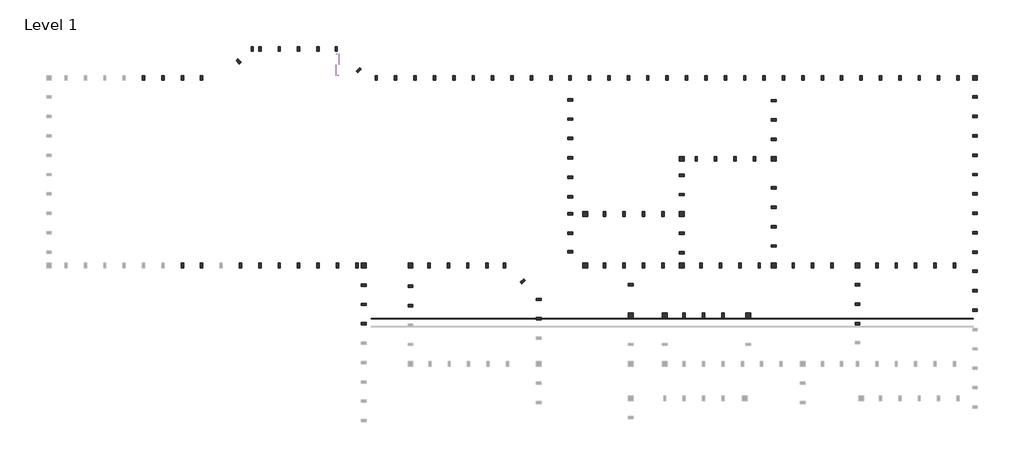
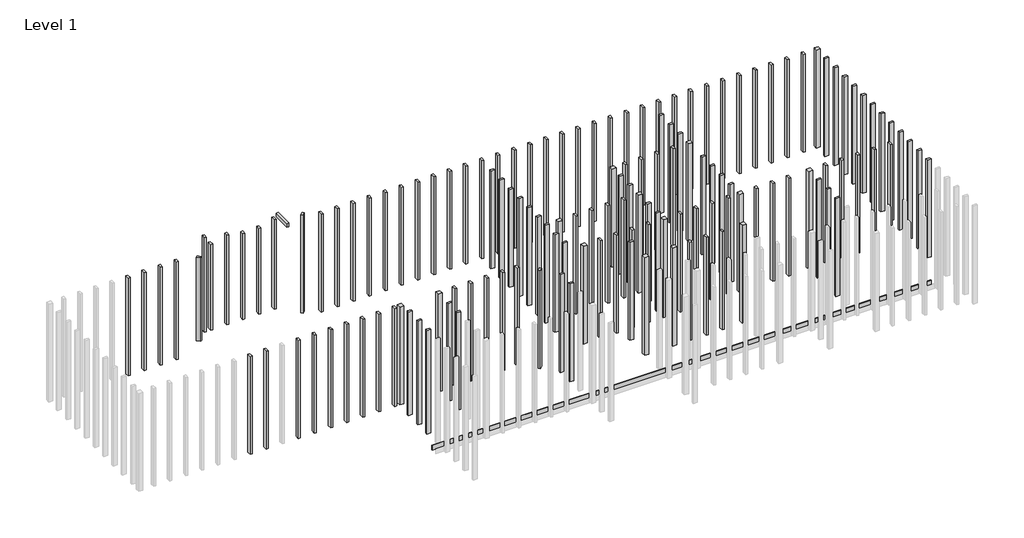
# One storey, part 2 of 2: 142 columns, 3 beams.
"""IFC4 building model written with IfcOpenShell, lengths in millimetres."""

import ifcopenshell
import ifcopenshell.guid

model = None  # the IFC model being written
_history = None  # IfcOwnerHistory: only IFC2X3 demands one
_inside = {}  # id of a spatial element -> (the spatial element, [elements in it])
_under = {}  # id of a project, library or spatial element -> (it, [spatial elements below it])
_declared = {}  # id of a project -> (the project, [libraries it declares])
_typed = {}  # id of a type object -> (the type object, [elements of that type])
_made_of = {}  # id of a material, layer set ... -> (it, [elements and type objects made of it])


def new_model(schema):
    """Start an empty IFC model of exactly this schema.

    Asked for "IFC4X3", IfcOpenShell would pick the latest addendum, in which some entities
    have other attributes; the version numbers below select the first issue.
    IFC2X3 requires an IfcOwnerHistory on every rooted entity: one is made here for all.
    """
    global model, _history
    if schema == "IFC4X3":
        model = ifcopenshell.file(schema_version=(4, 3, 0, 0))
    else:
        model = ifcopenshell.file(schema=schema)
    _inside.clear()
    _under.clear()
    _declared.clear()
    _typed.clear()
    _made_of.clear()
    _history = None
    if model.schema == "IFC2X3":
        org = make("IfcOrganization", Name="unknown")
        user = make(
            "IfcPersonAndOrganization",
            ThePerson=make("IfcPerson", FamilyName="unknown"),
            TheOrganization=org,
        )
        app = make(
            "IfcApplication",
            ApplicationDeveloper=org,
            Version="unknown",
            ApplicationFullName="unknown",
            ApplicationIdentifier="unknown",
        )
        _history = make(
            "IfcOwnerHistory",
            OwningUser=user,
            OwningApplication=app,
            ChangeAction="ADDED",
            CreationDate=0,
        )
    return model


def make(cls, **values):
    """One entity of the class cls with the attributes given. An attribute that is None is left unset."""
    return model.create_entity(
        cls, **{name: value for name, value in values.items() if value is not None}
    )


def rooted(cls, **values):
    """An entity with a GlobalId (a new one), such as an element, a storey or a relation."""
    return make(cls, GlobalId=ifcopenshell.guid.new(), OwnerHistory=_history, **values)


def si_unit(unit_type, name, prefix=None):
    """IfcSIUnit, for example si_unit("LENGTHUNIT", "METRE", prefix="MILLI")."""
    return make("IfcSIUnit", UnitType=unit_type, Prefix=prefix, Name=name)


def assignment(units):
    """IfcUnitAssignment: the units of a project."""
    return None if units is None else make("IfcUnitAssignment", Units=units)


def point(xyz):
    """IfcCartesianPoint."""
    return None if xyz is None else make("IfcCartesianPoint", Coordinates=xyz)


def direction(xyz):
    """IfcDirection."""
    return None if xyz is None else make("IfcDirection", DirectionRatios=xyz)


def frame(location, z_axis=None, x_axis=None):
    """IfcAxis2Placement3D, a coordinate frame: its origin and axes. An axis left out is left unset."""
    return make(
        "IfcAxis2Placement3D",
        Location=point(location),
        Axis=direction(z_axis),
        RefDirection=direction(x_axis),
    )


def origin():
    """The frame at (0, 0, 0) with its axes left unset."""
    return frame((0.0, 0.0, 0.0))


def origin_with_axes():
    """The frame at (0, 0, 0) with the z axis (0, 0, 1) and the x axis (1, 0, 0) written out."""
    return frame((0.0, 0.0, 0.0), z_axis=(0.0, 0.0, 1.0), x_axis=(1.0, 0.0, 0.0))


def place(relative_to, where):
    """IfcLocalPlacement: puts the frame where relative to a parent placement (None: the world)."""
    return make(
        "IfcLocalPlacement", PlacementRelTo=relative_to, RelativePlacement=where
    )


def context(
    kind, dimensions, precision=None, world=None, true_north=None, identifier=None
):
    """IfcGeometricRepresentationContext, for example the 3D "Model" context."""
    return make(
        "IfcGeometricRepresentationContext",
        ContextIdentifier=identifier,
        ContextType=kind,
        CoordinateSpaceDimension=dimensions,
        Precision=precision,
        WorldCoordinateSystem=world,
        TrueNorth=true_north,
    )


def project(units=None, contexts=None):
    """IfcProject with its units and contexts."""
    return rooted(
        "IfcProject",
        Name="project",
        RepresentationContexts=contexts,
        UnitsInContext=assignment(units),
    )


def spatial(cls, under=None, at=None, **own):
    """A site, building, storey or space (cls), placed at a placement, below another one or the project."""
    s = rooted(cls, ObjectPlacement=at, **own)
    if under is not None:
        _under.setdefault(under.id(), (under, []))[1].append(s)
    return s


def polyline(points):
    """IfcPolyline through the points."""
    return make("IfcPolyline", Points=[point(p) for p in points])


def outline(outer, holes=None, kind="AREA"):
    """IfcArbitraryClosedProfileDef: a profile drawn as a closed curve; with holes, ...WithVoids."""
    if holes is None:
        return make("IfcArbitraryClosedProfileDef", ProfileType=kind, OuterCurve=outer)
    return make(
        "IfcArbitraryProfileDefWithVoids",
        ProfileType=kind,
        OuterCurve=outer,
        InnerCurves=holes,
    )


def extrude(swept, where, along, depth):
    """IfcExtrudedAreaSolid: the profile swept, set in the frame where, extruded along a direction by depth."""
    return make(
        "IfcExtrudedAreaSolid",
        SweptArea=swept,
        Position=where,
        ExtrudedDirection=direction(along),
        Depth=depth,
    )


def shape(context_of_items, identifier, shape_type, items):
    """IfcShapeRepresentation: the items that make up one representation, for example the "Body"."""
    return make(
        "IfcShapeRepresentation",
        ContextOfItems=context_of_items,
        RepresentationIdentifier=identifier,
        RepresentationType=shape_type,
        Items=items,
    )


def source(mapping_origin, context_of_items, identifier, shape_type, items):
    """IfcRepresentationMap: a shape defined once, which mapped items show again and again."""
    return make(
        "IfcRepresentationMap",
        MappingOrigin=mapping_origin,
        MappedRepresentation=shape(context_of_items, identifier, shape_type, items),
    )


def transform(
    local_origin,
    x_axis=None,
    y_axis=None,
    z_axis=None,
    scale=None,
    scale2=None,
    scale3=None,
    uniform=True,
):
    """IfcCartesianTransformationOperator3D, or its non-uniform kind. x_axis, y_axis, z_axis: its Axis1, 2, 3."""
    if uniform:
        return make(
            "IfcCartesianTransformationOperator3D",
            Axis1=direction(x_axis),
            Axis2=direction(y_axis),
            LocalOrigin=point(local_origin),
            Scale=scale,
            Axis3=direction(z_axis),
        )
    return make(
        "IfcCartesianTransformationOperator3DnonUniform",
        Axis1=direction(x_axis),
        Axis2=direction(y_axis),
        LocalOrigin=point(local_origin),
        Scale=scale,
        Axis3=direction(z_axis),
        Scale2=scale2,
        Scale3=scale3,
    )


def mapped(mapping_source, mapping_target):
    """IfcMappedItem: shows the shape of a source again, moved by a transform."""
    return make(
        "IfcMappedItem", MappingSource=mapping_source, MappingTarget=mapping_target
    )


def made_of(thing, what):
    """Note that an element or type object is made of a material, layer set ...; save() writes the relation."""
    if what is not None:
        _made_of.setdefault(what.id(), (what, []))[1].append(thing)
    return thing


def element(
    cls,
    number,
    at=None,
    inside=None,
    cuts=None,
    type_object=None,
    material=None,
    context=None,
    identifier="Body",
    shape_type=None,
    held_by="IfcProductDefinitionShape",
    body=None,
    shapes=None,
    **own,
):
    """One element of the class cls, such as IfcWall. Its Tag is "e" and its number.

    at: its placement. inside: the storey or other place that contains it. cuts: it is an
    opening in that element (IfcRelVoidsElement). A single representation is given by context,
    identifier, shape_type and body (its items); several are given by shapes. held_by: the class
    of the entity that holds the representations. save() writes the other relations.
    """
    e = rooted(cls, Tag="e%d" % number, ObjectPlacement=at, **own)
    if body is not None:
        shapes = [shape(context, identifier, shape_type, body)]
    if shapes is not None:
        e.Representation = make(held_by, Representations=shapes)
    if inside is not None:
        _inside.setdefault(inside.id(), (inside, []))[1].append(e)
    if cuts is not None:
        rooted(
            "IfcRelVoidsElement", RelatingBuildingElement=cuts, RelatedOpeningElement=e
        )
    if type_object is not None:
        _typed.setdefault(type_object.id(), (type_object, []))[1].append(e)
    return made_of(e, material)


def aggregate(whole, parts):
    """IfcRelAggregates: a whole, such as a stair, and the parts it consists of."""
    return rooted("IfcRelAggregates", RelatingObject=whole, RelatedObjects=parts)


def save(model, path):
    """Write the relations noted so far, then the file.

    IfcRelAggregates (storeys below a building ...), IfcRelContainedInSpatialStructure (elements
    in a storey), IfcRelDefinesByType, IfcRelAssociatesMaterial and IfcRelDeclares: one each for
    every whole, place, type object, material and project.
    """
    for whole, parts in _under.values():
        aggregate(whole, parts)
    for where, things in _inside.values():
        rooted(
            "IfcRelContainedInSpatialStructure",
            RelatedElements=things,
            RelatingStructure=where,
        )
    for kind, things in _typed.values():
        rooted("IfcRelDefinesByType", RelatedObjects=things, RelatingType=kind)
    for what, things in _made_of.values():
        rooted("IfcRelAssociatesMaterial", RelatedObjects=things, RelatingMaterial=what)
    for by, libraries in _declared.values():
        rooted("IfcRelDeclares", RelatingContext=by, RelatedDefinitions=libraries)
    model.write(path)


def beam_b78a0881(model_context):
    return source(origin(), model_context, "Body", "SweptSolid", [
        extrude(outline(polyline([(228.6, 25.4), (228.6, -25.4), (-228.6, -25.4), (-228.6, 25.4), (228.6, 25.4)])), frame((0.0, 0.0, -50.8), z_axis=(0.0, 0.0, 1.0), x_axis=(1.0, 0.0, 0.0)), (0.0, 0.0, 1.0), 101.6),
    ])


def beam_af2566d3(model_context):
    return source(origin(), model_context, "Body", "SweptSolid", [
        extrude(outline(polyline([(6458.3020508, 5.55625), (6458.3020508, -5.55625), (-6159.1479492, -5.55625), (-6159.1479492, 5.55625), (6458.3020508, 5.55625)])), frame((0.0, 0.0, -63.5), z_axis=(0.0, 0.0, 1.0), x_axis=(1.0, 0.0, 0.0)), (0.0, 0.0, 1.0), 127.0),
    ])


def timber_column_65e54e3c(model_context):
    return source(origin(), model_context, "Body", "SweptSolid", [
        extrude(outline(polyline([(25.4, 50.8), (25.4, -50.8), (-25.4, -50.8), (-25.4, 50.8), (25.4, 50.8)])), frame((0.0, 0.0, 50.8), z_axis=(0.0, 0.0, 1.0), x_axis=(1.0, 0.0, 0.0)), (0.0, 0.0, 1.0), 2616.2),
    ])


def timber_column_b7e6a7b9(model_context):
    return source(origin(), model_context, "Body", "SweptSolid", [
        extrude(outline(polyline([(50.8, 50.8), (50.8, -50.8), (-50.8, -50.8), (-50.8, 50.8), (50.8, 50.8)])), frame((0.0, 0.0, 50.8), z_axis=(0.0, 0.0, 1.0), x_axis=(1.0, 0.0, 0.0)), (0.0, 0.0, 1.0), 2616.2),
    ])


def timber_column_c014de30(model_context):
    return source(origin(), model_context, "Body", "SweptSolid", [
        extrude(outline(polyline([(25.4, -50.8), (-25.4, -50.8), (-25.4, 50.8), (25.4, 50.8), (25.4, -50.8)])), frame((0.0, 0.0, 50.8), z_axis=(0.0, 0.0, 1.0), x_axis=(1.0, 0.0, 0.0)), (0.0, 0.0, 1.0), 2616.2),
    ])


def timber_column_7e99ce9a(model_context):
    return source(origin(), model_context, "Body", "SweptSolid", [
        extrude(outline(polyline([(25.4, 50.8), (25.4, -50.8), (-25.4, -50.8), (-25.4, 50.8), (25.4, 50.8)])), origin_with_axes(), (0.0, 0.0, 1.0), 2768.6),
    ])


def timber_column_b6a9144e(model_context):
    return source(origin(), model_context, "Body", "SweptSolid", [
        extrude(outline(polyline([(25.4, 50.8), (25.4, -50.8), (-25.4, -50.8), (-25.4, 50.8), (25.4, 50.8)])), frame((0.0, 0.0, 50.8), z_axis=(0.0, 0.0, 1.0), x_axis=(1.0, 0.0, 0.0)), (0.0, 0.0, 1.0), 2290.1727203),
    ])


model = new_model("IFC4")

# Units and contexts
model_context = context("Model", 3, world=origin())
ifc_project = project(units=[si_unit("LENGTHUNIT", "METRE", prefix="MILLI")], contexts=[model_context])

# Site, building, storey
site = spatial("IfcSite", under=ifc_project)
building = spatial("IfcBuilding", under=site)
storey = spatial("IfcBuildingStorey", under=building, Name="Level 1", Elevation=0.0)

# Beams
placement = place(None, origin())
beam_shape = beam_b78a0881(model_context)
element("IfcBeam", 1, ObjectType="Dimension Lumber : BLDG 6241 2X4\" TRUSS MEMBER", at=placement, inside=storey, context=model_context, shape_type="MappedRepresentation", body=[
    mapped(beam_shape, transform((-11705.214829, 5436.3284114, 2589.5072623), x_axis=(0.0, -1.0, 0.0), y_axis=(1.0, 0.0, 0.0), z_axis=(0.0, 0.0, 1.0))),
])
element("IfcBeam", 2, ObjectType="Dimension Lumber : BLDG 6241 2X4\" TRUSS MEMBER", at=placement, inside=storey, context=model_context, shape_type="MappedRepresentation", body=[
    mapped(beam_shape, transform((-11705.214829, 5436.3284114, 2589.5072623), x_axis=(0.0, -1.0, 0.0), y_axis=(1.0, 0.0, 0.0), z_axis=(0.0, 0.0, 1.0))),
])
beam_2_shape = beam_af2566d3(model_context)
element("IfcBeam", 3, ObjectType="Dimension Lumber : BLDG 6241 7/16\" Plywood Spacer", at=placement, inside=storey, context=model_context, shape_type="MappedRepresentation", body=[
    mapped(beam_2_shape, transform((-4542.0627783, 107.8846614, -510.38125), x_axis=(-1.0, 0.0, 0.0), y_axis=(0.0, -1.0, 0.0), z_axis=(0.0, 0.0, 1.0))),
])

# Columns
element("IfcColumn", 4, ObjectType="Timber-Column", at=placement, inside=storey, context=model_context, shape_type="SweptSolid", body=[
    extrude(outline(polyline([(-13305.414829, 5817.3284114), (-13305.414829, 5715.7284114), (-13356.214829, 5715.7284114), (-13356.214829, 5817.3284114), (-13305.414829, 5817.3284114)])), frame((0.0, 0.0, 50.8), z_axis=(0.0, 0.0, 1.0), x_axis=(1.0, 0.0, 0.0)), (0.0, 0.0, 1.0), 2290.1727203),
])
element("IfcColumn", 5, ObjectType="Timber-Column", at=placement, inside=storey, context=model_context, shape_type="SweptSolid", body=[
    extrude(outline(polyline([(-12899.014829, 5817.3284114), (-12899.014829, 5715.7284114), (-12949.814829, 5715.7284114), (-12949.814829, 5817.3284114), (-12899.014829, 5817.3284114)])), frame((0.0, 0.0, 50.8), z_axis=(0.0, 0.0, 1.0), x_axis=(1.0, 0.0, 0.0)), (0.0, 0.0, 1.0), 2391.7727203),
])
element("IfcColumn", 6, ObjectType="Timber-Column", at=placement, inside=storey, context=model_context, shape_type="SweptSolid", body=[
    extrude(outline(polyline([(-13793.9590772, 5557.3841632), (-13722.1170283, 5485.5421142), (-13758.0380528, 5449.6210897), (-13829.8801017, 5521.4631387), (-13793.9590772, 5557.3841632)])), frame((0.0, 0.0, 50.8), z_axis=(0.0, 0.0, 1.0), x_axis=(1.0, 0.0, 0.0)), (0.0, 0.0, 1.0), 2235.2),
])
element("IfcColumn", 7, ObjectType="Timber-Column", at=placement, inside=storey, context=model_context, shape_type="SweptSolid", body=[
    extrude(outline(polyline([(-13464.8030362, 5817.3284114), (-13464.8030362, 5715.7284114), (-13515.6030362, 5715.7284114), (-13515.6030362, 5817.3284114), (-13464.8030362, 5817.3284114)])), frame((0.0, 0.0, 50.8), z_axis=(0.0, 0.0, 1.0), x_axis=(1.0, 0.0, 0.0)), (0.0, 0.0, 1.0), 2528.0077467),
])
element("IfcColumn", 8, ObjectType="Timber-Column", at=placement, inside=storey, context=model_context, shape_type="SweptSolid", body=[
    extrude(outline(polyline([(-11705.214829, 5817.3284114), (-11705.214829, 5715.7284114), (-11756.014829, 5715.7284114), (-11756.014829, 5817.3284114), (-11705.214829, 5817.3284114)])), frame((0.0, 0.0, 50.8), z_axis=(0.0, 0.0, 1.0), x_axis=(1.0, 0.0, 0.0)), (0.0, 0.0, 1.0), 2391.7727203),
])
timber_column_shape = timber_column_65e54e3c(model_context)
element("IfcColumn", 9, ObjectType="Timber-Column", at=placement, inside=storey, context=model_context, shape_type="MappedRepresentation", body=[
    mapped(timber_column_shape, transform((-15769.214829, 5156.9284114, 0.0), x_axis=(1.0, 0.0, 0.0), y_axis=(0.0, 1.0, 0.0), z_axis=(0.0, 0.0, 1.0))),
])
element("IfcColumn", 10, ObjectType="Timber-Column", at=placement, inside=storey, context=model_context, shape_type="MappedRepresentation", body=[
    mapped(timber_column_shape, transform((-15362.814829, 5156.9284114, 0.0), x_axis=(1.0, 0.0, 0.0), y_axis=(0.0, 1.0, 0.0), z_axis=(0.0, 0.0, 1.0))),
])
element("IfcColumn", 11, ObjectType="Timber-Column", at=placement, inside=storey, context=model_context, shape_type="MappedRepresentation", body=[
    mapped(timber_column_shape, transform((-14956.414829, 5156.9284114, 0.0), x_axis=(1.0, 0.0, 0.0), y_axis=(0.0, 1.0, 0.0), z_axis=(0.0, 0.0, 1.0))),
])
element("IfcColumn", 12, ObjectType="Timber-Column", at=placement, inside=storey, context=model_context, shape_type="MappedRepresentation", body=[
    mapped(timber_column_shape, transform((-14550.014829, 5156.9284114, 0.0), x_axis=(1.0, 0.0, 0.0), y_axis=(0.0, 1.0, 0.0), z_axis=(0.0, 0.0, 1.0))),
])
element("IfcColumn", 13, ObjectType="Timber-Column", at=placement, inside=storey, context=model_context, shape_type="MappedRepresentation", body=[
    mapped(timber_column_shape, transform((-10892.414829, 5156.9284114, 0.0), x_axis=(1.0, 0.0, 0.0), y_axis=(0.0, 1.0, 0.0), z_axis=(0.0, 0.0, 1.0))),
])
element("IfcColumn", 14, ObjectType="Timber-Column", at=placement, inside=storey, context=model_context, shape_type="MappedRepresentation", body=[
    mapped(timber_column_shape, transform((-10486.014829, 5156.9284114, 0.0), x_axis=(1.0, 0.0, 0.0), y_axis=(0.0, 1.0, 0.0), z_axis=(0.0, 0.0, 1.0))),
])
element("IfcColumn", 15, ObjectType="Timber-Column", at=placement, inside=storey, context=model_context, shape_type="MappedRepresentation", body=[
    mapped(timber_column_shape, transform((-10079.614829, 5156.9284114, 0.0), x_axis=(1.0, 0.0, 0.0), y_axis=(0.0, 1.0, 0.0), z_axis=(0.0, 0.0, 1.0))),
])
element("IfcColumn", 16, ObjectType="Timber-Column", at=placement, inside=storey, context=model_context, shape_type="MappedRepresentation", body=[
    mapped(timber_column_shape, transform((-9673.214829, 5156.9284114, 0.0), x_axis=(1.0, 0.0, 0.0), y_axis=(0.0, 1.0, 0.0), z_axis=(0.0, 0.0, 1.0))),
])
element("IfcColumn", 17, ObjectType="Timber-Column", at=placement, inside=storey, context=model_context, shape_type="MappedRepresentation", body=[
    mapped(timber_column_shape, transform((-9266.814829, 5156.9284114, 0.0), x_axis=(1.0, 0.0, 0.0), y_axis=(0.0, 1.0, 0.0), z_axis=(0.0, 0.0, 1.0))),
])
element("IfcColumn", 18, ObjectType="Timber-Column", at=placement, inside=storey, context=model_context, shape_type="MappedRepresentation", body=[
    mapped(timber_column_shape, transform((-8860.414829, 5156.9284114, 0.0), x_axis=(1.0, 0.0, 0.0), y_axis=(0.0, 1.0, 0.0), z_axis=(0.0, 0.0, 1.0))),
])
element("IfcColumn", 19, ObjectType="Timber-Column", at=placement, inside=storey, context=model_context, shape_type="MappedRepresentation", body=[
    mapped(timber_column_shape, transform((-8454.014829, 5156.9284114, 0.0), x_axis=(1.0, 0.0, 0.0), y_axis=(0.0, 1.0, 0.0), z_axis=(0.0, 0.0, 1.0))),
])
element("IfcColumn", 20, ObjectType="Timber-Column", at=placement, inside=storey, context=model_context, shape_type="MappedRepresentation", body=[
    mapped(timber_column_shape, transform((-8047.614829, 5156.9284114, 0.0), x_axis=(1.0, 0.0, 0.0), y_axis=(0.0, 1.0, 0.0), z_axis=(0.0, 0.0, 1.0))),
])
element("IfcColumn", 21, ObjectType="Timber-Column", at=placement, inside=storey, context=model_context, shape_type="MappedRepresentation", body=[
    mapped(timber_column_shape, transform((-7641.214829, 5156.9284114, 0.0), x_axis=(1.0, 0.0, 0.0), y_axis=(0.0, 1.0, 0.0), z_axis=(0.0, 0.0, 1.0))),
])
element("IfcColumn", 22, ObjectType="Timber-Column", at=placement, inside=storey, context=model_context, shape_type="MappedRepresentation", body=[
    mapped(timber_column_shape, transform((-7234.814829, 5156.9284114, 0.0), x_axis=(1.0, 0.0, 0.0), y_axis=(0.0, 1.0, 0.0), z_axis=(0.0, 0.0, 1.0))),
])
element("IfcColumn", 23, ObjectType="Timber-Column", at=placement, inside=storey, context=model_context, shape_type="MappedRepresentation", body=[
    mapped(timber_column_shape, transform((-6828.414829, 5156.9284114, 0.0), x_axis=(1.0, 0.0, 0.0), y_axis=(0.0, 1.0, 0.0), z_axis=(0.0, 0.0, 1.0))),
])
element("IfcColumn", 24, ObjectType="Timber-Column", at=placement, inside=storey, context=model_context, shape_type="MappedRepresentation", body=[
    mapped(timber_column_shape, transform((-6422.014829, 5156.9284114, 0.0), x_axis=(1.0, 0.0, 0.0), y_axis=(0.0, 1.0, 0.0), z_axis=(0.0, 0.0, 1.0))),
])
element("IfcColumn", 25, ObjectType="Timber-Column", at=placement, inside=storey, context=model_context, shape_type="MappedRepresentation", body=[
    mapped(timber_column_shape, transform((-6015.614829, 5156.9284114, 0.0), x_axis=(1.0, 0.0, 0.0), y_axis=(0.0, 1.0, 0.0), z_axis=(0.0, 0.0, 1.0))),
])
element("IfcColumn", 26, ObjectType="Timber-Column", at=placement, inside=storey, context=model_context, shape_type="MappedRepresentation", body=[
    mapped(timber_column_shape, transform((-5609.214829, 5156.9284114, 0.0), x_axis=(1.0, 0.0, 0.0), y_axis=(0.0, 1.0, 0.0), z_axis=(0.0, 0.0, 1.0))),
])
element("IfcColumn", 27, ObjectType="Timber-Column", at=placement, inside=storey, context=model_context, shape_type="MappedRepresentation", body=[
    mapped(timber_column_shape, transform((-5202.814829, 5156.9284114, 0.0), x_axis=(1.0, 0.0, 0.0), y_axis=(0.0, 1.0, 0.0), z_axis=(0.0, 0.0, 1.0))),
])
element("IfcColumn", 28, ObjectType="Timber-Column", at=placement, inside=storey, context=model_context, shape_type="MappedRepresentation", body=[
    mapped(timber_column_shape, transform((-4796.414829, 5156.9284114, 0.0), x_axis=(1.0, 0.0, 0.0), y_axis=(0.0, 1.0, 0.0), z_axis=(0.0, 0.0, 1.0))),
])
element("IfcColumn", 29, ObjectType="Timber-Column", at=placement, inside=storey, context=model_context, shape_type="MappedRepresentation", body=[
    mapped(timber_column_shape, transform((-4390.014829, 5156.9284114, 0.0), x_axis=(1.0, 0.0, 0.0), y_axis=(0.0, 1.0, 0.0), z_axis=(0.0, 0.0, 1.0))),
])
element("IfcColumn", 30, ObjectType="Timber-Column", at=placement, inside=storey, context=model_context, shape_type="MappedRepresentation", body=[
    mapped(timber_column_shape, transform((-3983.614829, 5156.9284114, 0.0), x_axis=(1.0, 0.0, 0.0), y_axis=(0.0, 1.0, 0.0), z_axis=(0.0, 0.0, 1.0))),
])
element("IfcColumn", 31, ObjectType="Timber-Column", at=placement, inside=storey, context=model_context, shape_type="MappedRepresentation", body=[
    mapped(timber_column_shape, transform((-3577.214829, 5156.9284114, 0.0), x_axis=(1.0, 0.0, 0.0), y_axis=(0.0, 1.0, 0.0), z_axis=(0.0, 0.0, 1.0))),
])
element("IfcColumn", 32, ObjectType="Timber-Column", at=placement, inside=storey, context=model_context, shape_type="MappedRepresentation", body=[
    mapped(timber_column_shape, transform((-3170.814829, 5156.9284114, 0.0), x_axis=(1.0, 0.0, 0.0), y_axis=(0.0, 1.0, 0.0), z_axis=(0.0, 0.0, 1.0))),
])
element("IfcColumn", 33, ObjectType="Timber-Column", at=placement, inside=storey, context=model_context, shape_type="MappedRepresentation", body=[
    mapped(timber_column_shape, transform((-2764.414829, 5156.9284114, 0.0), x_axis=(1.0, 0.0, 0.0), y_axis=(0.0, 1.0, 0.0), z_axis=(0.0, 0.0, 1.0))),
])
element("IfcColumn", 34, ObjectType="Timber-Column", at=placement, inside=storey, context=model_context, shape_type="MappedRepresentation", body=[
    mapped(timber_column_shape, transform((-2358.014829, 5156.9284114, 0.0), x_axis=(1.0, 0.0, 0.0), y_axis=(0.0, 1.0, 0.0), z_axis=(0.0, 0.0, 1.0))),
])
element("IfcColumn", 35, ObjectType="Timber-Column", at=placement, inside=storey, context=model_context, shape_type="MappedRepresentation", body=[
    mapped(timber_column_shape, transform((-1951.614829, 5156.9284114, 0.0), x_axis=(1.0, 0.0, 0.0), y_axis=(0.0, 1.0, 0.0), z_axis=(0.0, 0.0, 1.0))),
])
element("IfcColumn", 36, ObjectType="Timber-Column", at=placement, inside=storey, context=model_context, shape_type="MappedRepresentation", body=[
    mapped(timber_column_shape, transform((-1545.214829, 5156.9284114, 0.0), x_axis=(1.0, 0.0, 0.0), y_axis=(0.0, 1.0, 0.0), z_axis=(0.0, 0.0, 1.0))),
])
element("IfcColumn", 37, ObjectType="Timber-Column", at=placement, inside=storey, context=model_context, shape_type="MappedRepresentation", body=[
    mapped(timber_column_shape, transform((-1138.814829, 5156.9284114, 0.0), x_axis=(1.0, 0.0, 0.0), y_axis=(0.0, 1.0, 0.0), z_axis=(0.0, 0.0, 1.0))),
])
element("IfcColumn", 38, ObjectType="Timber-Column", at=placement, inside=storey, context=model_context, shape_type="MappedRepresentation", body=[
    mapped(timber_column_shape, transform((-732.414829, 5156.9284114, 0.0), x_axis=(1.0, 0.0, 0.0), y_axis=(0.0, 1.0, 0.0), z_axis=(0.0, 0.0, 1.0))),
])
element("IfcColumn", 39, ObjectType="Timber-Column", at=placement, inside=storey, context=model_context, shape_type="MappedRepresentation", body=[
    mapped(timber_column_shape, transform((-326.014829, 5156.9284114, 0.0), x_axis=(1.0, 0.0, 0.0), y_axis=(0.0, 1.0, 0.0), z_axis=(0.0, 0.0, 1.0))),
])
element("IfcColumn", 40, ObjectType="Timber-Column", at=placement, inside=storey, context=model_context, shape_type="MappedRepresentation", body=[
    mapped(timber_column_shape, transform((80.385171, 5156.9284114, 0.0), x_axis=(1.0, 0.0, 0.0), y_axis=(0.0, 1.0, 0.0), z_axis=(0.0, 0.0, 1.0))),
])
element("IfcColumn", 41, ObjectType="Timber-Column", at=placement, inside=storey, context=model_context, shape_type="MappedRepresentation", body=[
    mapped(timber_column_shape, transform((486.785171, 5156.9284114, 0.0), x_axis=(1.0, 0.0, 0.0), y_axis=(0.0, 1.0, 0.0), z_axis=(0.0, 0.0, 1.0))),
])
element("IfcColumn", 42, ObjectType="Timber-Column", at=placement, inside=storey, context=model_context, shape_type="MappedRepresentation", body=[
    mapped(timber_column_shape, transform((893.185171, 5156.9284114, 0.0), x_axis=(1.0, 0.0, 0.0), y_axis=(0.0, 1.0, 0.0), z_axis=(0.0, 0.0, 1.0))),
])
element("IfcColumn", 43, ObjectType="Timber-Column", at=placement, inside=storey, context=model_context, shape_type="MappedRepresentation", body=[
    mapped(timber_column_shape, transform((1299.585171, 5156.9284114, 0.0), x_axis=(1.0, 0.0, 0.0), y_axis=(0.0, 1.0, 0.0), z_axis=(0.0, 0.0, 1.0))),
])
element("IfcColumn", 44, ObjectType="Timber-Column", at=placement, inside=storey, context=model_context, shape_type="MappedRepresentation", body=[
    mapped(timber_column_shape, transform((-11298.814829, 1226.2784114, 0.0), x_axis=(1.0, 0.0, 0.0), y_axis=(0.0, 1.0, 0.0), z_axis=(0.0, 0.0, 1.0))),
])
element("IfcColumn", 45, ObjectType="Timber-Column", at=placement, inside=storey, context=model_context, shape_type="MappedRepresentation", body=[
    mapped(timber_column_shape, transform((-11705.214829, 1226.2784114, 0.0), x_axis=(1.0, 0.0, 0.0), y_axis=(0.0, 1.0, 0.0), z_axis=(0.0, 0.0, 1.0))),
])
element("IfcColumn", 46, ObjectType="Timber-Column", at=placement, inside=storey, context=model_context, shape_type="MappedRepresentation", body=[
    mapped(timber_column_shape, transform((-12111.614829, 1226.2784114, 0.0), x_axis=(1.0, 0.0, 0.0), y_axis=(0.0, 1.0, 0.0), z_axis=(0.0, 0.0, 1.0))),
])
element("IfcColumn", 47, ObjectType="Timber-Column", at=placement, inside=storey, context=model_context, shape_type="MappedRepresentation", body=[
    mapped(timber_column_shape, transform((-12518.014829, 1226.2784114, 0.0), x_axis=(1.0, 0.0, 0.0), y_axis=(0.0, 1.0, 0.0), z_axis=(0.0, 0.0, 1.0))),
])
element("IfcColumn", 48, ObjectType="Timber-Column", at=placement, inside=storey, context=model_context, shape_type="MappedRepresentation", body=[
    mapped(timber_column_shape, transform((-12924.414829, 1226.2784114, 0.0), x_axis=(1.0, 0.0, 0.0), y_axis=(0.0, 1.0, 0.0), z_axis=(0.0, 0.0, 1.0))),
])
element("IfcColumn", 49, ObjectType="Timber-Column", at=placement, inside=storey, context=model_context, shape_type="MappedRepresentation", body=[
    mapped(timber_column_shape, transform((-13330.814829, 1226.2784114, 0.0), x_axis=(1.0, 0.0, 0.0), y_axis=(0.0, 1.0, 0.0), z_axis=(0.0, 0.0, 1.0))),
])
element("IfcColumn", 50, ObjectType="Timber-Column", at=placement, inside=storey, context=model_context, shape_type="MappedRepresentation", body=[
    mapped(timber_column_shape, transform((-13737.214829, 1226.2784114, 0.0), x_axis=(1.0, 0.0, 0.0), y_axis=(0.0, 1.0, 0.0), z_axis=(0.0, 0.0, 1.0))),
])
element("IfcColumn", 51, ObjectType="Timber-Column", at=placement, inside=storey, context=model_context, shape_type="MappedRepresentation", body=[
    mapped(timber_column_shape, transform((-14550.014829, 1226.2784114, 0.0), x_axis=(1.0, 0.0, 0.0), y_axis=(0.0, 1.0, 0.0), z_axis=(0.0, 0.0, 1.0))),
])
element("IfcColumn", 52, ObjectType="Timber-Column", at=placement, inside=storey, context=model_context, shape_type="MappedRepresentation", body=[
    mapped(timber_column_shape, transform((-14956.414829, 1226.2784114, 0.0), x_axis=(1.0, 0.0, 0.0), y_axis=(0.0, 1.0, 0.0), z_axis=(0.0, 0.0, 1.0))),
])
element("IfcColumn", 53, ObjectType="Timber-Column", at=placement, inside=storey, context=model_context, shape_type="MappedRepresentation", body=[
    mapped(timber_column_shape, transform((-11259.6474151, 5320.9609974, 0.0), x_axis=(0.7071067811865546, -0.7071067811865406, 0.0), y_axis=(0.7071067811865406, 0.7071067811865546, 0.0), z_axis=(0.0, 0.0, 1.0))),
])
element("IfcColumn", 54, ObjectType="Timber-Column", at=placement, inside=storey, context=model_context, shape_type="MappedRepresentation", body=[
    mapped(timber_column_shape, transform((-6828.414829, 4699.7284114, 0.0), x_axis=(0.0, 1.0, 0.0), y_axis=(-1.0, 0.0, 0.0), z_axis=(0.0, 0.0, 1.0))),
])
element("IfcColumn", 55, ObjectType="Timber-Column", at=placement, inside=storey, context=model_context, shape_type="MappedRepresentation", body=[
    mapped(timber_column_shape, transform((-6828.414829, 4293.3284114, 0.0), x_axis=(0.0, 1.0, 0.0), y_axis=(-1.0, 0.0, 0.0), z_axis=(0.0, 0.0, 1.0))),
])
element("IfcColumn", 56, ObjectType="Timber-Column", at=placement, inside=storey, context=model_context, shape_type="MappedRepresentation", body=[
    mapped(timber_column_shape, transform((-6828.414829, 3886.9284114, 0.0), x_axis=(0.0, 1.0, 0.0), y_axis=(-1.0, 0.0, 0.0), z_axis=(0.0, 0.0, 1.0))),
])
element("IfcColumn", 57, ObjectType="Timber-Column", at=placement, inside=storey, context=model_context, shape_type="MappedRepresentation", body=[
    mapped(timber_column_shape, transform((-6828.414829, 3480.5284114, 0.0), x_axis=(0.0, 1.0, 0.0), y_axis=(-1.0, 0.0, 0.0), z_axis=(0.0, 0.0, 1.0))),
])
element("IfcColumn", 58, ObjectType="Timber-Column", at=placement, inside=storey, context=model_context, shape_type="MappedRepresentation", body=[
    mapped(timber_column_shape, transform((-6828.414829, 3074.1284114, 0.0), x_axis=(0.0, 1.0, 0.0), y_axis=(-1.0, 0.0, 0.0), z_axis=(0.0, 0.0, 1.0))),
])
element("IfcColumn", 59, ObjectType="Timber-Column", at=placement, inside=storey, context=model_context, shape_type="MappedRepresentation", body=[
    mapped(timber_column_shape, transform((-6828.414829, 2667.7284114, 0.0), x_axis=(0.0, 1.0, 0.0), y_axis=(-1.0, 0.0, 0.0), z_axis=(0.0, 0.0, 1.0))),
])
element("IfcColumn", 60, ObjectType="Timber-Column", at=placement, inside=storey, context=model_context, shape_type="MappedRepresentation", body=[
    mapped(timber_column_shape, transform((-6828.414829, 2305.7784114, 0.0), x_axis=(0.0, 1.0, 0.0), y_axis=(-1.0, 0.0, 0.0), z_axis=(0.0, 0.0, 1.0))),
])
element("IfcColumn", 61, ObjectType="Timber-Column", at=placement, inside=storey, context=model_context, shape_type="MappedRepresentation", body=[
    mapped(timber_column_shape, transform((-6828.414829, 1899.3784114, 0.0), x_axis=(0.0, 1.0, 0.0), y_axis=(-1.0, 0.0, 0.0), z_axis=(0.0, 0.0, 1.0))),
])
element("IfcColumn", 62, ObjectType="Timber-Column", at=placement, inside=storey, context=model_context, shape_type="MappedRepresentation", body=[
    mapped(timber_column_shape, transform((-6828.414829, 1516.0125093, 0.0), x_axis=(0.0, 1.0, 0.0), y_axis=(-1.0, 0.0, 0.0), z_axis=(0.0, 0.0, 1.0))),
])
element("IfcColumn", 63, ObjectType="Timber-Column", at=placement, inside=storey, context=model_context, shape_type="MappedRepresentation", body=[
    mapped(timber_column_shape, transform((-6106.8807311, 1226.2784114, 0.0), x_axis=(-1.0, 0.0, 0.0), y_axis=(0.0, -1.0, 0.0), z_axis=(0.0, 0.0, 1.0))),
])
element("IfcColumn", 64, ObjectType="Timber-Column", at=placement, inside=storey, context=model_context, shape_type="MappedRepresentation", body=[
    mapped(timber_column_shape, transform((-5700.4807311, 1226.2784114, 0.0), x_axis=(-1.0, 0.0, 0.0), y_axis=(0.0, -1.0, 0.0), z_axis=(0.0, 0.0, 1.0))),
])
element("IfcColumn", 65, ObjectType="Timber-Column", at=placement, inside=storey, context=model_context, shape_type="MappedRepresentation", body=[
    mapped(timber_column_shape, transform((-5294.0807311, 1226.2784114, 0.0), x_axis=(-1.0, 0.0, 0.0), y_axis=(0.0, -1.0, 0.0), z_axis=(0.0, 0.0, 1.0))),
])
element("IfcColumn", 66, ObjectType="Timber-Column", at=placement, inside=storey, context=model_context, shape_type="MappedRepresentation", body=[
    mapped(timber_column_shape, transform((-4887.6807311, 1226.2784114, 0.0), x_axis=(-1.0, 0.0, 0.0), y_axis=(0.0, -1.0, 0.0), z_axis=(0.0, 0.0, 1.0))),
])
element("IfcColumn", 67, ObjectType="Timber-Column", at=placement, inside=storey, context=model_context, shape_type="MappedRepresentation", body=[
    mapped(timber_column_shape, transform((-4085.214829, 1226.2784114, 0.0), x_axis=(-1.0, 0.0, 0.0), y_axis=(0.0, -1.0, 0.0), z_axis=(0.0, 0.0, 1.0))),
])
element("IfcColumn", 68, ObjectType="Timber-Column", at=placement, inside=storey, context=model_context, shape_type="MappedRepresentation", body=[
    mapped(timber_column_shape, transform((-3678.814829, 1226.2784114, 0.0), x_axis=(-1.0, 0.0, 0.0), y_axis=(0.0, -1.0, 0.0), z_axis=(0.0, 0.0, 1.0))),
])
element("IfcColumn", 69, ObjectType="Timber-Column", at=placement, inside=storey, context=model_context, shape_type="MappedRepresentation", body=[
    mapped(timber_column_shape, transform((-3272.414829, 1226.2784114, 0.0), x_axis=(-1.0, 0.0, 0.0), y_axis=(0.0, -1.0, 0.0), z_axis=(0.0, 0.0, 1.0))),
])
element("IfcColumn", 70, ObjectType="Timber-Column", at=placement, inside=storey, context=model_context, shape_type="MappedRepresentation", body=[
    mapped(timber_column_shape, transform((-2866.014829, 1226.2784114, 0.0), x_axis=(-1.0, 0.0, 0.0), y_axis=(0.0, -1.0, 0.0), z_axis=(0.0, 0.0, 1.0))),
])
element("IfcColumn", 71, ObjectType="Timber-Column", at=placement, inside=storey, context=model_context, shape_type="MappedRepresentation", body=[
    mapped(timber_column_shape, transform((-2154.814829, 1226.2784114, 0.0), x_axis=(-1.0, 0.0, 0.0), y_axis=(0.0, -1.0, 0.0), z_axis=(0.0, 0.0, 1.0))),
])
element("IfcColumn", 72, ObjectType="Timber-Column", at=placement, inside=storey, context=model_context, shape_type="MappedRepresentation", body=[
    mapped(timber_column_shape, transform((-1748.414829, 1226.2784114, 0.0), x_axis=(-1.0, 0.0, 0.0), y_axis=(0.0, -1.0, 0.0), z_axis=(0.0, 0.0, 1.0))),
])
element("IfcColumn", 73, ObjectType="Timber-Column", at=placement, inside=storey, context=model_context, shape_type="MappedRepresentation", body=[
    mapped(timber_column_shape, transform((-1342.014829, 1226.2784114, 0.0), x_axis=(-1.0, 0.0, 0.0), y_axis=(0.0, -1.0, 0.0), z_axis=(0.0, 0.0, 1.0))),
])
element("IfcColumn", 74, ObjectType="Timber-Column", at=placement, inside=storey, context=model_context, shape_type="MappedRepresentation", body=[
    mapped(timber_column_shape, transform((-402.214829, 1226.2784114, 0.0), x_axis=(-1.0, 0.0, 0.0), y_axis=(0.0, -1.0, 0.0), z_axis=(0.0, 0.0, 1.0))),
])
element("IfcColumn", 75, ObjectType="Timber-Column", at=placement, inside=storey, context=model_context, shape_type="MappedRepresentation", body=[
    mapped(timber_column_shape, transform((4.185171, 1226.2784114, 0.0), x_axis=(-1.0, 0.0, 0.0), y_axis=(0.0, -1.0, 0.0), z_axis=(0.0, 0.0, 1.0))),
])
element("IfcColumn", 76, ObjectType="Timber-Column", at=placement, inside=storey, context=model_context, shape_type="MappedRepresentation", body=[
    mapped(timber_column_shape, transform((410.585171, 1226.2784114, 0.0), x_axis=(-1.0, 0.0, 0.0), y_axis=(0.0, -1.0, 0.0), z_axis=(0.0, 0.0, 1.0))),
])
element("IfcColumn", 77, ObjectType="Timber-Column", at=placement, inside=storey, context=model_context, shape_type="MappedRepresentation", body=[
    mapped(timber_column_shape, transform((816.985171, 1226.2784114, 0.0), x_axis=(-1.0, 0.0, 0.0), y_axis=(0.0, -1.0, 0.0), z_axis=(0.0, 0.0, 1.0))),
])
element("IfcColumn", 78, ObjectType="Timber-Column", at=placement, inside=storey, context=model_context, shape_type="MappedRepresentation", body=[
    mapped(timber_column_shape, transform((1223.385171, 1226.2784114, 0.0), x_axis=(-1.0, 0.0, 0.0), y_axis=(0.0, -1.0, 0.0), z_axis=(0.0, 0.0, 1.0))),
])
element("IfcColumn", 79, ObjectType="Timber-Column", at=placement, inside=storey, context=model_context, shape_type="MappedRepresentation", body=[
    mapped(timber_column_shape, transform((-6106.8807311, 2305.7784114, 0.0), x_axis=(-1.0, 0.0, 0.0), y_axis=(0.0, -1.0, 0.0), z_axis=(0.0, 0.0, 1.0))),
])
element("IfcColumn", 80, ObjectType="Timber-Column", at=placement, inside=storey, context=model_context, shape_type="MappedRepresentation", body=[
    mapped(timber_column_shape, transform((-5700.4807311, 2305.7784114, 0.0), x_axis=(-1.0, 0.0, 0.0), y_axis=(0.0, -1.0, 0.0), z_axis=(0.0, 0.0, 1.0))),
])
element("IfcColumn", 81, ObjectType="Timber-Column", at=placement, inside=storey, context=model_context, shape_type="MappedRepresentation", body=[
    mapped(timber_column_shape, transform((-5294.0807311, 2305.7784114, 0.0), x_axis=(-1.0, 0.0, 0.0), y_axis=(0.0, -1.0, 0.0), z_axis=(0.0, 0.0, 1.0))),
])
element("IfcColumn", 82, ObjectType="Timber-Column", at=placement, inside=storey, context=model_context, shape_type="MappedRepresentation", body=[
    mapped(timber_column_shape, transform((-4887.6807311, 2305.7784114, 0.0), x_axis=(-1.0, 0.0, 0.0), y_axis=(0.0, -1.0, 0.0), z_axis=(0.0, 0.0, 1.0))),
])
element("IfcColumn", 83, ObjectType="Timber-Column", at=placement, inside=storey, context=model_context, shape_type="MappedRepresentation", body=[
    mapped(timber_column_shape, transform((-4491.614829, 1899.3784114, 0.0), x_axis=(0.0, 1.0, 0.0), y_axis=(-1.0, 0.0, 0.0), z_axis=(0.0, 0.0, 1.0))),
])
element("IfcColumn", 84, ObjectType="Timber-Column", at=placement, inside=storey, context=model_context, shape_type="MappedRepresentation", body=[
    mapped(timber_column_shape, transform((-4491.614829, 1492.9784114, 0.0), x_axis=(0.0, 1.0, 0.0), y_axis=(-1.0, 0.0, 0.0), z_axis=(0.0, 0.0, 1.0))),
])
element("IfcColumn", 85, ObjectType="Timber-Column", at=placement, inside=storey, context=model_context, shape_type="MappedRepresentation", body=[
    mapped(timber_column_shape, transform((-4491.614829, 2712.1784114, 0.0), x_axis=(0.0, 1.0, 0.0), y_axis=(-1.0, 0.0, 0.0), z_axis=(0.0, 0.0, 1.0))),
])
element("IfcColumn", 86, ObjectType="Timber-Column", at=placement, inside=storey, context=model_context, shape_type="MappedRepresentation", body=[
    mapped(timber_column_shape, transform((-4491.614829, 3118.5784114, 0.0), x_axis=(0.0, 1.0, 0.0), y_axis=(-1.0, 0.0, 0.0), z_axis=(0.0, 0.0, 1.0))),
])
element("IfcColumn", 87, ObjectType="Timber-Column", at=placement, inside=storey, context=model_context, shape_type="MappedRepresentation", body=[
    mapped(timber_column_shape, transform((-2967.614829, 3461.4784114, 0.0), x_axis=(1.0, 0.0, 0.0), y_axis=(0.0, 1.0, 0.0), z_axis=(0.0, 0.0, 1.0))),
])
element("IfcColumn", 88, ObjectType="Timber-Column", at=placement, inside=storey, context=model_context, shape_type="MappedRepresentation", body=[
    mapped(timber_column_shape, transform((-3374.014829, 3461.4784114, 0.0), x_axis=(1.0, 0.0, 0.0), y_axis=(0.0, 1.0, 0.0), z_axis=(0.0, 0.0, 1.0))),
])
element("IfcColumn", 89, ObjectType="Timber-Column", at=placement, inside=storey, context=model_context, shape_type="MappedRepresentation", body=[
    mapped(timber_column_shape, transform((-3780.414829, 3461.4784114, 0.0), x_axis=(1.0, 0.0, 0.0), y_axis=(0.0, 1.0, 0.0), z_axis=(0.0, 0.0, 1.0))),
])
element("IfcColumn", 90, ObjectType="Timber-Column", at=placement, inside=storey, context=model_context, shape_type="MappedRepresentation", body=[
    mapped(timber_column_shape, transform((-4186.814829, 3461.4784114, 0.0), x_axis=(1.0, 0.0, 0.0), y_axis=(0.0, 1.0, 0.0), z_axis=(0.0, 0.0, 1.0))),
])
element("IfcColumn", 91, ObjectType="Timber-Column", at=placement, inside=storey, context=model_context, shape_type="MappedRepresentation", body=[
    mapped(timber_column_shape, transform((-2561.214829, 1632.6784114, 0.0), x_axis=(0.0, 1.0, 0.0), y_axis=(-1.0, 0.0, 0.0), z_axis=(0.0, 0.0, 1.0))),
])
element("IfcColumn", 92, ObjectType="Timber-Column", at=placement, inside=storey, context=model_context, shape_type="MappedRepresentation", body=[
    mapped(timber_column_shape, transform((-2561.214829, 2039.0784114, 0.0), x_axis=(0.0, 1.0, 0.0), y_axis=(-1.0, 0.0, 0.0), z_axis=(0.0, 0.0, 1.0))),
])
element("IfcColumn", 93, ObjectType="Timber-Column", at=placement, inside=storey, context=model_context, shape_type="MappedRepresentation", body=[
    mapped(timber_column_shape, transform((-2561.214829, 2445.4784114, 0.0), x_axis=(0.0, 1.0, 0.0), y_axis=(-1.0, 0.0, 0.0), z_axis=(0.0, 0.0, 1.0))),
])
element("IfcColumn", 94, ObjectType="Timber-Column", at=placement, inside=storey, context=model_context, shape_type="MappedRepresentation", body=[
    mapped(timber_column_shape, transform((-2561.214829, 2851.8784114, 0.0), x_axis=(0.0, 1.0, 0.0), y_axis=(-1.0, 0.0, 0.0), z_axis=(0.0, 0.0, 1.0))),
])
element("IfcColumn", 95, ObjectType="Timber-Column", at=placement, inside=storey, context=model_context, shape_type="MappedRepresentation", body=[
    mapped(timber_column_shape, transform((-8203.998927, 1226.2784114, 0.0), x_axis=(1.0, 0.0, 0.0), y_axis=(0.0, 1.0, 0.0), z_axis=(0.0, 0.0, 1.0))),
])
element("IfcColumn", 96, ObjectType="Timber-Column", at=placement, inside=storey, context=model_context, shape_type="MappedRepresentation", body=[
    mapped(timber_column_shape, transform((-8568.7720585, 1226.2784114, 0.0), x_axis=(1.0, 0.0, 0.0), y_axis=(0.0, 1.0, 0.0), z_axis=(0.0, 0.0, 1.0))),
])
element("IfcColumn", 97, ObjectType="Timber-Column", at=placement, inside=storey, context=model_context, shape_type="MappedRepresentation", body=[
    mapped(timber_column_shape, transform((-8975.1720585, 1226.2784114, 0.0), x_axis=(1.0, 0.0, 0.0), y_axis=(0.0, 1.0, 0.0), z_axis=(0.0, 0.0, 1.0))),
])
element("IfcColumn", 98, ObjectType="Timber-Column", at=placement, inside=storey, context=model_context, shape_type="MappedRepresentation", body=[
    mapped(timber_column_shape, transform((-9381.5720585, 1226.2784114, 0.0), x_axis=(1.0, 0.0, 0.0), y_axis=(0.0, 1.0, 0.0), z_axis=(0.0, 0.0, 1.0))),
])
element("IfcColumn", 99, ObjectType="Timber-Column", at=placement, inside=storey, context=model_context, shape_type="MappedRepresentation", body=[
    mapped(timber_column_shape, transform((-9787.9720585, 1226.2784114, 0.0), x_axis=(1.0, 0.0, 0.0), y_axis=(0.0, 1.0, 0.0), z_axis=(0.0, 0.0, 1.0))),
])
element("IfcColumn", 100, ObjectType="Timber-Column", at=placement, inside=storey, context=model_context, shape_type="MappedRepresentation", body=[
    mapped(timber_column_shape, transform((-7488.814829, 511.0943134, 0.0), x_axis=(0.0, 1.0, 0.0), y_axis=(-1.0, 0.0, 0.0), z_axis=(0.0, 0.0, 1.0))),
])
element("IfcColumn", 101, ObjectType="Timber-Column", at=placement, inside=storey, context=model_context, shape_type="MappedRepresentation", body=[
    mapped(timber_column_shape, transform((-7488.814829, 104.6943134, 0.0), x_axis=(0.0, 1.0, 0.0), y_axis=(-1.0, 0.0, 0.0), z_axis=(0.0, 0.0, 1.0))),
])
element("IfcColumn", 102, ObjectType="Timber-Column", at=placement, inside=storey, context=model_context, shape_type="MappedRepresentation", body=[
    mapped(timber_column_shape, transform((-7822.589312, 891.3108454, 0.0), x_axis=(0.7071067811865449, -0.70710678118655, 0.0), y_axis=(0.70710678118655, 0.7071067811865449, 0.0), z_axis=(0.0, 0.0, 1.0))),
])
element("IfcColumn", 103, ObjectType="Timber-Column", at=placement, inside=storey, context=model_context, shape_type="MappedRepresentation", body=[
    mapped(timber_column_shape, transform((-2561.214829, 3867.8784114, 0.0), x_axis=(0.0, 1.0, 0.0), y_axis=(-1.0, 0.0, 0.0), z_axis=(0.0, 0.0, 1.0))),
])
element("IfcColumn", 104, ObjectType="Timber-Column", at=placement, inside=storey, context=model_context, shape_type="MappedRepresentation", body=[
    mapped(timber_column_shape, transform((-2561.214829, 4274.2784114, 0.0), x_axis=(0.0, 1.0, 0.0), y_axis=(-1.0, 0.0, 0.0), z_axis=(0.0, 0.0, 1.0))),
])
element("IfcColumn", 105, ObjectType="Timber-Column", at=placement, inside=storey, context=model_context, shape_type="MappedRepresentation", body=[
    mapped(timber_column_shape, transform((-2561.214829, 4680.6784114, 0.0), x_axis=(0.0, 1.0, 0.0), y_axis=(-1.0, 0.0, 0.0), z_axis=(0.0, 0.0, 1.0))),
])
element("IfcColumn", 106, ObjectType="Timber-Column", at=placement, inside=storey, context=model_context, shape_type="MappedRepresentation", body=[
    mapped(timber_column_shape, transform((-10175.1225949, 381.7284114, 0.0), x_axis=(0.0, 1.0, 0.0), y_axis=(-1.0, 0.0, 0.0), z_axis=(0.0, 0.0, 1.0))),
])
element("IfcColumn", 107, ObjectType="Timber-Column", at=placement, inside=storey, context=model_context, shape_type="MappedRepresentation", body=[
    mapped(timber_column_shape, transform((-10175.1225949, 788.1284114, 0.0), x_axis=(0.0, 1.0, 0.0), y_axis=(-1.0, 0.0, 0.0), z_axis=(0.0, 0.0, 1.0))),
])
element("IfcColumn", 108, ObjectType="Timber-Column", at=placement, inside=storey, context=model_context, shape_type="MappedRepresentation", body=[
    mapped(timber_column_shape, transform((-5558.414829, 819.8784114, 0.0), x_axis=(0.0, 1.0, 0.0), y_axis=(-1.0, 0.0, 0.0), z_axis=(0.0, 0.0, 1.0))),
])
element("IfcColumn", 109, ObjectType="Timber-Column", at=placement, inside=storey, context=model_context, shape_type="MappedRepresentation", body=[
    mapped(timber_column_shape, transform((-4440.814829, 178.5284114, 0.0), x_axis=(-1.0, 0.0, 0.0), y_axis=(0.0, -1.0, 0.0), z_axis=(0.0, 0.0, 1.0))),
])
element("IfcColumn", 110, ObjectType="Timber-Column", at=placement, inside=storey, context=model_context, shape_type="MappedRepresentation", body=[
    mapped(timber_column_shape, transform((-4034.414829, 178.5284114, 0.0), x_axis=(-1.0, 0.0, 0.0), y_axis=(0.0, -1.0, 0.0), z_axis=(0.0, 0.0, 1.0))),
])
element("IfcColumn", 111, ObjectType="Timber-Column", at=placement, inside=storey, context=model_context, shape_type="MappedRepresentation", body=[
    mapped(timber_column_shape, transform((-3628.014829, 178.5284114, 0.0), x_axis=(-1.0, 0.0, 0.0), y_axis=(0.0, -1.0, 0.0), z_axis=(0.0, 0.0, 1.0))),
])
element("IfcColumn", 112, ObjectType="Timber-Column", at=placement, inside=storey, context=model_context, shape_type="MappedRepresentation", body=[
    mapped(timber_column_shape, transform((-808.614829, 819.8784114, 0.0), x_axis=(0.0, 1.0, 0.0), y_axis=(-1.0, 0.0, 0.0), z_axis=(0.0, 0.0, 1.0))),
])
element("IfcColumn", 113, ObjectType="Timber-Column", at=placement, inside=storey, context=model_context, shape_type="MappedRepresentation", body=[
    mapped(timber_column_shape, transform((-808.614829, 413.4784114, 0.0), x_axis=(0.0, 1.0, 0.0), y_axis=(-1.0, 0.0, 0.0), z_axis=(0.0, 0.0, 1.0))),
])
element("IfcColumn", 114, ObjectType="Timber-Column", at=placement, inside=storey, context=model_context, shape_type="MappedRepresentation", body=[
    mapped(timber_column_shape, transform((-808.614829, 7.0784114, 0.0), x_axis=(0.0, 1.0, 0.0), y_axis=(-1.0, 0.0, 0.0), z_axis=(0.0, 0.0, 1.0))),
])
timber_column_2_shape = timber_column_b7e6a7b9(model_context)
element("IfcColumn", 115, ObjectType="Timber-Column", at=placement, inside=storey, context=model_context, shape_type="MappedRepresentation", body=[
    mapped(timber_column_2_shape, transform((-11152.764829, 1226.2784114, 0.0), x_axis=(1.0, 0.0, 0.0), y_axis=(0.0, 1.0, 0.0), z_axis=(0.0, 0.0, 1.0))),
])
element("IfcColumn", 116, ObjectType="Timber-Column", at=placement, inside=storey, context=model_context, shape_type="MappedRepresentation", body=[
    mapped(timber_column_2_shape, transform((1655.185171, 5156.9284114, 0.0), x_axis=(1.0, 0.0, 0.0), y_axis=(0.0, 1.0, 0.0), z_axis=(0.0, 0.0, 1.0))),
])
element("IfcColumn", 117, ObjectType="Timber-Column", at=placement, inside=storey, context=model_context, shape_type="MappedRepresentation", body=[
    mapped(timber_column_2_shape, transform((-4491.614829, 3461.4784114, 0.0), x_axis=(1.0, 0.0, 0.0), y_axis=(0.0, 1.0, 0.0), z_axis=(0.0, 0.0, 1.0))),
])
element("IfcColumn", 118, ObjectType="Timber-Column", at=placement, inside=storey, context=model_context, shape_type="MappedRepresentation", body=[
    mapped(timber_column_2_shape, transform((-4491.614829, 2305.7784114, 0.0), x_axis=(1.0, 0.0, 0.0), y_axis=(0.0, 1.0, 0.0), z_axis=(0.0, 0.0, 1.0))),
])
element("IfcColumn", 119, ObjectType="Timber-Column", at=placement, inside=storey, context=model_context, shape_type="MappedRepresentation", body=[
    mapped(timber_column_2_shape, transform((-4491.614829, 1226.2784114, 0.0), x_axis=(1.0, 0.0, 0.0), y_axis=(0.0, 1.0, 0.0), z_axis=(0.0, 0.0, 1.0))),
])
element("IfcColumn", 120, ObjectType="Timber-Column", at=placement, inside=storey, context=model_context, shape_type="MappedRepresentation", body=[
    mapped(timber_column_2_shape, transform((-2561.214829, 1226.2784114, 0.0), x_axis=(1.0, 0.0, 0.0), y_axis=(0.0, 1.0, 0.0), z_axis=(0.0, 0.0, 1.0))),
])
element("IfcColumn", 121, ObjectType="Timber-Column", at=placement, inside=storey, context=model_context, shape_type="MappedRepresentation", body=[
    mapped(timber_column_2_shape, transform((-2561.214829, 3461.4784114, 0.0), x_axis=(1.0, 0.0, 0.0), y_axis=(0.0, 1.0, 0.0), z_axis=(0.0, 0.0, 1.0))),
])
element("IfcColumn", 122, ObjectType="Timber-Column", at=placement, inside=storey, context=model_context, shape_type="MappedRepresentation", body=[
    mapped(timber_column_2_shape, transform((-6513.2807311, 1226.2784114, 0.0), x_axis=(1.0, 0.0, 0.0), y_axis=(0.0, 1.0, 0.0), z_axis=(0.0, 0.0, 1.0))),
])
element("IfcColumn", 123, ObjectType="Timber-Column", at=placement, inside=storey, context=model_context, shape_type="MappedRepresentation", body=[
    mapped(timber_column_2_shape, transform((-6513.2807311, 2305.7784114, 0.0), x_axis=(1.0, 0.0, 0.0), y_axis=(0.0, 1.0, 0.0), z_axis=(0.0, 0.0, 1.0))),
])
element("IfcColumn", 124, ObjectType="Timber-Column", at=placement, inside=storey, context=model_context, shape_type="MappedRepresentation", body=[
    mapped(timber_column_2_shape, transform((-808.614829, 1226.2784114, 0.0), x_axis=(1.0, 0.0, 0.0), y_axis=(0.0, 1.0, 0.0), z_axis=(0.0, 0.0, 1.0))),
])
element("IfcColumn", 125, ObjectType="Timber-Column", at=placement, inside=storey, context=model_context, shape_type="MappedRepresentation", body=[
    mapped(timber_column_2_shape, transform((-5558.414829, 178.5284114, 0.0), x_axis=(1.0, 0.0, 0.0), y_axis=(0.0, 1.0, 0.0), z_axis=(0.0, 0.0, 1.0))),
])
element("IfcColumn", 126, ObjectType="Timber-Column", at=placement, inside=storey, context=model_context, shape_type="MappedRepresentation", body=[
    mapped(timber_column_2_shape, transform((-10174.864829, 1226.2784114, 0.0), x_axis=(1.0, 0.0, 0.0), y_axis=(0.0, 1.0, 0.0), z_axis=(0.0, 0.0, 1.0))),
])
element("IfcColumn", 127, ObjectType="Timber-Column", at=placement, inside=storey, context=model_context, shape_type="MappedRepresentation", body=[
    mapped(timber_column_2_shape, transform((-3094.614829, 178.5284114, 0.0), x_axis=(1.0, 0.0, 0.0), y_axis=(0.0, 1.0, 0.0), z_axis=(0.0, 0.0, 1.0))),
])
element("IfcColumn", 128, ObjectType="Timber-Column", at=placement, inside=storey, context=model_context, shape_type="MappedRepresentation", body=[
    mapped(timber_column_2_shape, transform((-4847.214829, 178.5284114, 0.0), x_axis=(1.0, 0.0, 0.0), y_axis=(0.0, 1.0, 0.0), z_axis=(0.0, 0.0, 1.0))),
])
timber_column_3_shape = timber_column_c014de30(model_context)
element("IfcColumn", 129, ObjectType="Timber-Column", at=placement, inside=storey, context=model_context, shape_type="MappedRepresentation", body=[
    mapped(timber_column_3_shape, transform((1655.185171, 4756.8784114, 0.0), x_axis=(0.0, 1.0, 0.0), y_axis=(-1.0, 0.0, 0.0), z_axis=(0.0, 0.0, 1.0))),
])
element("IfcColumn", 130, ObjectType="Timber-Column", at=placement, inside=storey, context=model_context, shape_type="MappedRepresentation", body=[
    mapped(timber_column_3_shape, transform((1655.185171, 4350.4784114, 0.0), x_axis=(0.0, 1.0, 0.0), y_axis=(-1.0, 0.0, 0.0), z_axis=(0.0, 0.0, 1.0))),
])
element("IfcColumn", 131, ObjectType="Timber-Column", at=placement, inside=storey, context=model_context, shape_type="MappedRepresentation", body=[
    mapped(timber_column_3_shape, transform((1655.185171, 3944.0784114, 0.0), x_axis=(0.0, 1.0, 0.0), y_axis=(-1.0, 0.0, 0.0), z_axis=(0.0, 0.0, 1.0))),
])
element("IfcColumn", 132, ObjectType="Timber-Column", at=placement, inside=storey, context=model_context, shape_type="MappedRepresentation", body=[
    mapped(timber_column_3_shape, transform((1655.185171, 3537.6784114, 0.0), x_axis=(0.0, 1.0, 0.0), y_axis=(-1.0, 0.0, 0.0), z_axis=(0.0, 0.0, 1.0))),
])
element("IfcColumn", 133, ObjectType="Timber-Column", at=placement, inside=storey, context=model_context, shape_type="MappedRepresentation", body=[
    mapped(timber_column_3_shape, transform((1655.185171, 3131.2784114, 0.0), x_axis=(0.0, 1.0, 0.0), y_axis=(-1.0, 0.0, 0.0), z_axis=(0.0, 0.0, 1.0))),
])
element("IfcColumn", 134, ObjectType="Timber-Column", at=placement, inside=storey, context=model_context, shape_type="MappedRepresentation", body=[
    mapped(timber_column_3_shape, transform((1655.185171, 2724.8784114, 0.0), x_axis=(0.0, 1.0, 0.0), y_axis=(-1.0, 0.0, 0.0), z_axis=(0.0, 0.0, 1.0))),
])
element("IfcColumn", 135, ObjectType="Timber-Column", at=placement, inside=storey, context=model_context, shape_type="MappedRepresentation", body=[
    mapped(timber_column_3_shape, transform((1655.185171, 2318.4784114, 0.0), x_axis=(0.0, 1.0, 0.0), y_axis=(-1.0, 0.0, 0.0), z_axis=(0.0, 0.0, 1.0))),
])
element("IfcColumn", 136, ObjectType="Timber-Column", at=placement, inside=storey, context=model_context, shape_type="MappedRepresentation", body=[
    mapped(timber_column_3_shape, transform((1655.185171, 1912.0784114, 0.0), x_axis=(0.0, 1.0, 0.0), y_axis=(-1.0, 0.0, 0.0), z_axis=(0.0, 0.0, 1.0))),
])
element("IfcColumn", 137, ObjectType="Timber-Column", at=placement, inside=storey, context=model_context, shape_type="MappedRepresentation", body=[
    mapped(timber_column_3_shape, transform((1655.185171, 1505.6784114, 0.0), x_axis=(0.0, 1.0, 0.0), y_axis=(-1.0, 0.0, 0.0), z_axis=(0.0, 0.0, 1.0))),
])
element("IfcColumn", 138, ObjectType="Timber-Column", at=placement, inside=storey, context=model_context, shape_type="MappedRepresentation", body=[
    mapped(timber_column_3_shape, transform((1655.185171, 1099.2784114, 0.0), x_axis=(0.0, 1.0, 0.0), y_axis=(-1.0, 0.0, 0.0), z_axis=(0.0, 0.0, 1.0))),
])
element("IfcColumn", 139, ObjectType="Timber-Column", at=placement, inside=storey, context=model_context, shape_type="MappedRepresentation", body=[
    mapped(timber_column_3_shape, transform((1655.185171, 692.8784114, 0.0), x_axis=(0.0, 1.0, 0.0), y_axis=(-1.0, 0.0, 0.0), z_axis=(0.0, 0.0, 1.0))),
])
element("IfcColumn", 140, ObjectType="Timber-Column", at=placement, inside=storey, context=model_context, shape_type="MappedRepresentation", body=[
    mapped(timber_column_3_shape, transform((1655.185171, 286.4784114, 0.0), x_axis=(0.0, 1.0, 0.0), y_axis=(-1.0, 0.0, 0.0), z_axis=(0.0, 0.0, 1.0))),
])
timber_column_4_shape = timber_column_7e99ce9a(model_context)
element("IfcColumn", 141, ObjectType="Timber-Column", at=placement, inside=storey, context=model_context, shape_type="MappedRepresentation", body=[
    mapped(timber_column_4_shape, transform((-11152.764829, 813.5284114, 0.0), x_axis=(0.0, 1.0, 0.0), y_axis=(-1.0, 0.0, 0.0), z_axis=(0.0, 0.0, 1.0))),
])
element("IfcColumn", 142, ObjectType="Timber-Column", at=placement, inside=storey, context=model_context, shape_type="MappedRepresentation", body=[
    mapped(timber_column_4_shape, transform((-11152.764829, 407.1284114, 0.0), x_axis=(0.0, 1.0, 0.0), y_axis=(-1.0, 0.0, 0.0), z_axis=(0.0, 0.0, 1.0))),
])
element("IfcColumn", 143, ObjectType="Timber-Column", at=placement, inside=storey, context=model_context, shape_type="MappedRepresentation", body=[
    mapped(timber_column_4_shape, transform((-11152.764829, 0.7284114, 0.0), x_axis=(0.0, 1.0, 0.0), y_axis=(-1.0, 0.0, 0.0), z_axis=(0.0, 0.0, 1.0))),
])
timber_column_5_shape = timber_column_b6a9144e(model_context)
element("IfcColumn", 144, ObjectType="Timber-Column", at=placement, inside=storey, context=model_context, shape_type="MappedRepresentation", body=[
    mapped(timber_column_5_shape, transform((-12518.014829, 5766.5284114, 0.0), x_axis=(1.0, 0.0, 0.0), y_axis=(0.0, 1.0, 0.0), z_axis=(0.0, 0.0, 1.0))),
])
element("IfcColumn", 145, ObjectType="Timber-Column", at=placement, inside=storey, context=model_context, shape_type="MappedRepresentation", body=[
    mapped(timber_column_5_shape, transform((-12111.614829, 5766.5284114, 0.0), x_axis=(1.0, 0.0, 0.0), y_axis=(0.0, 1.0, 0.0), z_axis=(0.0, 0.0, 1.0))),
])

save(model, "model.ifc")

# Revit data of these elements
# Type "Dimension Lumber : BLDG 6241 2X4\" TRUSS MEMBER"
#   Assembly Code = "B10"
#   A = 0.273472 SF
#   Length [instance default] = 5' - 0"
#   b = 0' - 2"
#   d = 0' - 4"
#   Structural Material [instance default] = Softwood, Lumber
# Type "Dimension Lumber : BLDG 6241 7/16\" Plywood Spacer"
#   Assembly Code = "B10"
#   A = 0.273472 SF
#   Length [instance default] = 5' - 0"
#   b = 0' - 0 7/16"
#   d = 0' - 5"
#   Structural Material [instance default] = Softwood, Lumber
# Type "Timber-Column : BLDG 6241 Wall Struds 2\"x4\""
#   Assembly Code = "B10"
#   A = 0.140625 SF
#   b = 0' - 2"
#   d = 0' - 4"
#   Structural Material [instance default] = Softwood, Lumber
# Type "Timber-Column : BLDG 6241 Wall Struds 4\"x4\""
#   Assembly Code = "B10"
#   A = 0.140625 SF
#   b = 0' - 4"
#   d = 0' - 4"
#   Structural Material [instance default] = Softwood, Lumber
# Elements 1, 2 (IfcBeam, "Dimension Lumber : BLDG 6241 2X4\" TRUSS MEMBER")
#   Comments = ""
#   Structural Material = Softwood, Lumber
#   Phase Created = New Construction
#   Materials on its faces: "Softwood, Lumber"
# Element 3 (IfcBeam, "Dimension Lumber : BLDG 6241 7/16\" Plywood Spacer")
#   Comments = ""
#   Structural Material = Plywood, Sheathing
#   Phase Created = New Construction
#   Materials on its faces: "Plywood, Sheathing"
